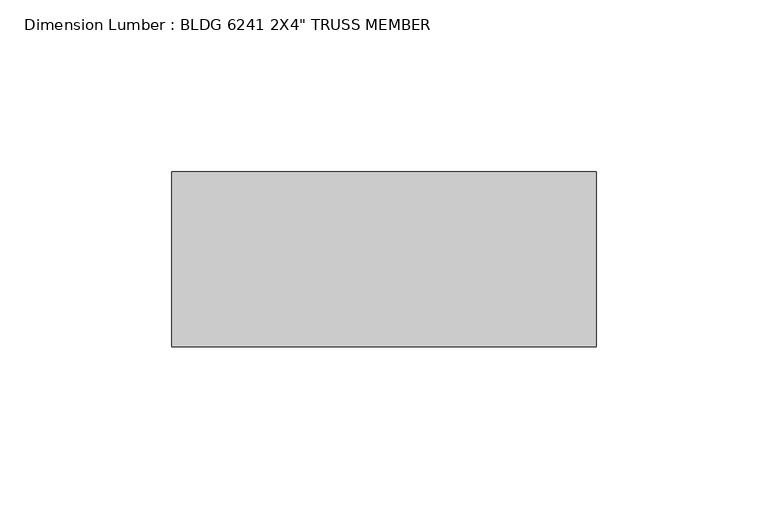
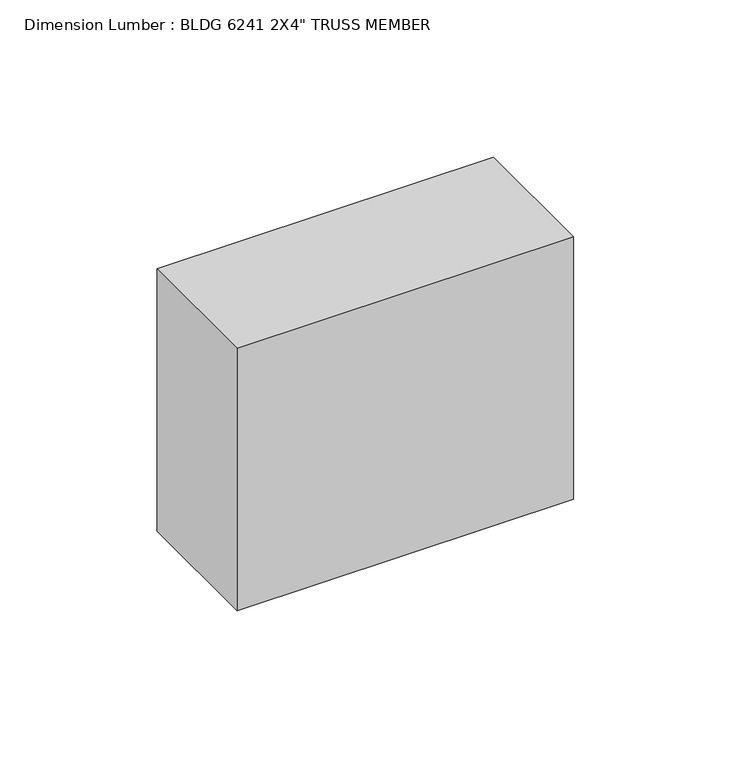
"""IFC4 building model written with IfcOpenShell, lengths in millimetres: beam geometry."""

from ifc_helpers import new_model, si_unit, frame, origin, place, context, project, spatial, polyline, outline, extrude, source, transform, mapped, element, save


def beam_dfed05dc(model_context):
    return source(origin(), model_context, "Body", "SweptSolid", [
        extrude(outline(polyline([(63.8057136, -25.4), (-59.553433, -25.4), (-59.553433, 25.4), (63.8057136, 25.4), (63.8057136, -25.4)])), frame((0.0, 0.0, -50.8), z_axis=(0.0, 0.0, 1.0), x_axis=(1.0, 0.0, 0.0)), (0.0, 0.0, 1.0), 101.6),
    ])


if __name__ == "__main__":
    model = new_model("IFC4")
    model_context = context("Model", 3, world=origin())
    ifc_project = project(units=[si_unit("LENGTHUNIT", "METRE", prefix="MILLI")], contexts=[model_context])
    site = spatial("IfcSite", under=ifc_project)
    building = spatial("IfcBuilding", under=site)
    placement = place(None, origin())
    beam_shape = beam_dfed05dc(model_context)
    element("IfcBeam", 1, ObjectType="Dimension Lumber : BLDG 6241 2X4\" TRUSS MEMBER", at=placement, inside=building, context=model_context, shape_type="MappedRepresentation", body=[
        mapped(beam_shape, transform((0.0, 0.0, 0.0), x_axis=(1.0, 0.0, 0.0), y_axis=(0.0, 1.0, 0.0), z_axis=(0.0, 0.0, 1.0))),
    ])
    save(model, "model.ifc")

# Revit data of these elements
# Type "Dimension Lumber : BLDG 6241 2X4\" TRUSS MEMBER"
#   Assembly Code = "B10"
#   A = 0.273472 SF
#   Length [instance default] = 5' - 0"
#   b = 0' - 2"
#   d = 0' - 4"
#   Structural Material [instance default] = Softwood, Lumber
# Element 1 (IfcBeam, "Dimension Lumber : BLDG 6241 2X4\" TRUSS MEMBER")
#   Materials on its faces: "Softwood, Lumber"
# Materials
#   "Softwood, Lumber": class "Wood", colour RGB 223 192 134, transparency 0, Description = "Pinus Echinata", Cost = 0
